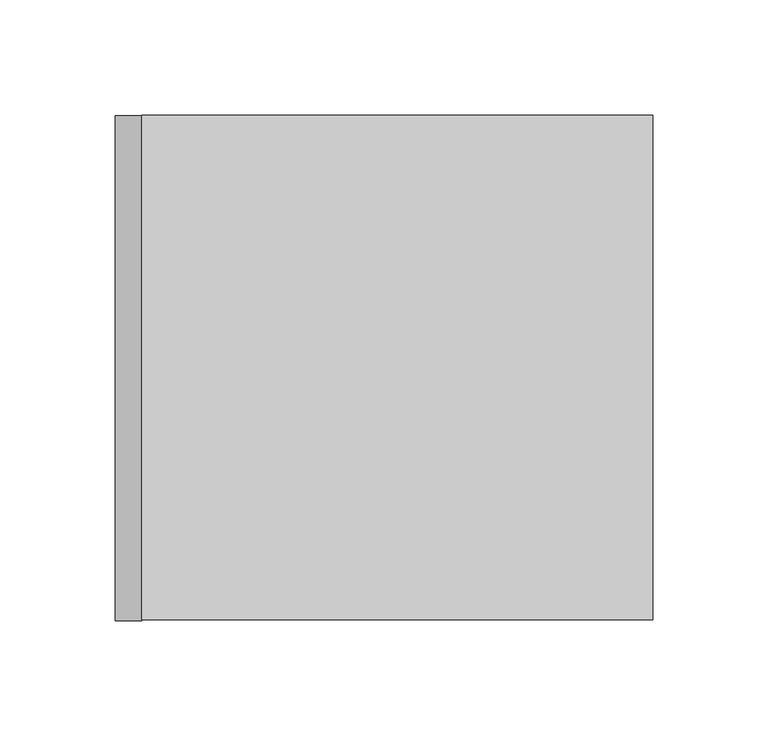
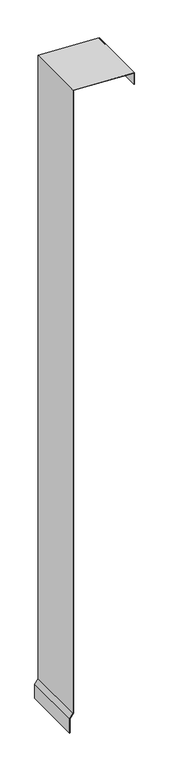
"""IFC4 building model written with IfcOpenShell, lengths in millimetres: proxy geometry, Generic Models 7:Generic Models 1:5:Generic Models 1:5 : Generic Models 7:Generic Models 1:337419:11 : Generic Models 7:Generic Models 1:5:Generic Models 1:5 : Generic Models 7:Generic Models 1:337419:311462."""

from ifc_helpers import new_model, si_unit, frame, origin, place, context, project, spatial, polyline, outline, extrude, source, transform, mapped, element, save


def generic_models_f6a12301(model_context):
    return source(origin(), model_context, "Body", "SweptSolid", [
        extrude(outline(polyline([(3795.8885169, 560352.1679739), (6178.9388113, 560352.1679739), (6167.4563403, 560571.2665711), (6125.115987, 560571.2665711), (6125.115987, 560572.8540711), (6168.9628216, 560572.8540711), (6180.6116872, 560350.5804739), (3796.3890538, 560350.5804739), (3779.8619698, 560339.0080851), (3725.3283058, 560339.0080851), (3725.3283058, 560340.5955851), (3779.361433, 560340.5955851), (3795.8885169, 560352.1679739)])), frame((0.0, -579015.7726341, 0.0), z_axis=(0.0, 1.0, 0.0), x_axis=(0.0, 0.0, 1.0)), (0.0, 0.0, 1.0), 219.4960882),
    ])


if __name__ == "__main__":
    model = new_model("IFC4")
    model_context = context("Model", 3, world=origin())
    ifc_project = project(units=[si_unit("LENGTHUNIT", "METRE", prefix="MILLI")], contexts=[model_context])
    site = spatial("IfcSite", under=ifc_project)
    building = spatial("IfcBuilding", under=site)
    placement = place(None, origin())
    generic_models_shape = generic_models_f6a12301(model_context)
    element("IfcBuildingElementProxy", 1, Name="Generic Models 7:Generic Models 1:5:Generic Models 1:5 : Generic Models 7:Generic Models 1:337419:11 : Generic Models 7:Generic Models 1:5:Generic Models 1:5 : Generic Models 7:Generic Models 1:337419:311462", ObjectType="Generic Models 7:Generic Models 1:5:Generic Models 1:5 : Generic Models 7:Generic Models 1:337419:11 : Generic Models 7:Generic Models 1:5:Generic Models 1:5 : Generic Models 7:Generic Models 1:337419:311462", at=placement, inside=building, context=model_context, shape_type="MappedRepresentation", body=[
        mapped(generic_models_shape, transform((0.0, 0.0, 0.0), x_axis=(1.0, 0.0, 0.0), y_axis=(0.0, 1.0, 0.0), z_axis=(0.0, 0.0, 1.0))),
    ])
    save(model, "model.ifc")

# Revit data of these elements
# Type "Generic Models 7:Generic Models 1:5:Generic Models 1:5 : Generic Models 7:Generic Models 1:337419:11 : Generic Models 7:Generic Models 1:5:Generic Models 1:5 : Generic Models 7:Generic Models 1:337419:311462"
#   NameOverride = "Generic Models 7:Generic Models 1:5:Generic Models 1:5 : Generic Models 7:Generic Models 1:337419:311462"
#   ObjectTypeOverride = "Generic Models 1:5 : Generic Models 7:Generic Models 1:337419"
#   Reference = "Generic Models 1"
#   Tag = "311462"
# Element 1 (IfcBuildingElementProxy, "Generic Models 7:Generic Models 1:5:Generic Models 1:5 : Generic Models 7:Generic Models 1:337419:11 : Generic Models 7:Generic Models 1:5:Generic Models 1:5 : Generic Models 7:Generic Models 1:337419:311462")
#   Materials on its faces: "UV STABLE WATER RESISTANT VAPOR PERMEABLE AIR BARRIER (WRB) - WRAP JAMBS/HEADERS - BLACK COLOR"
# Materials
#   "UV STABLE WATER RESISTANT VAPOR PERMEABLE AIR BARRIER (WRB) - WRAP JAMBS/HEADERS - BLACK COLOR": class "Generic", colour RGB 51 162 45, transparency 0, Description = "Polyethylene film membrane", Cost = 0
